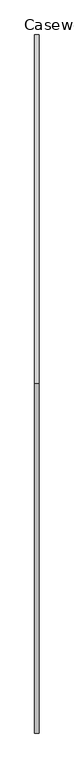
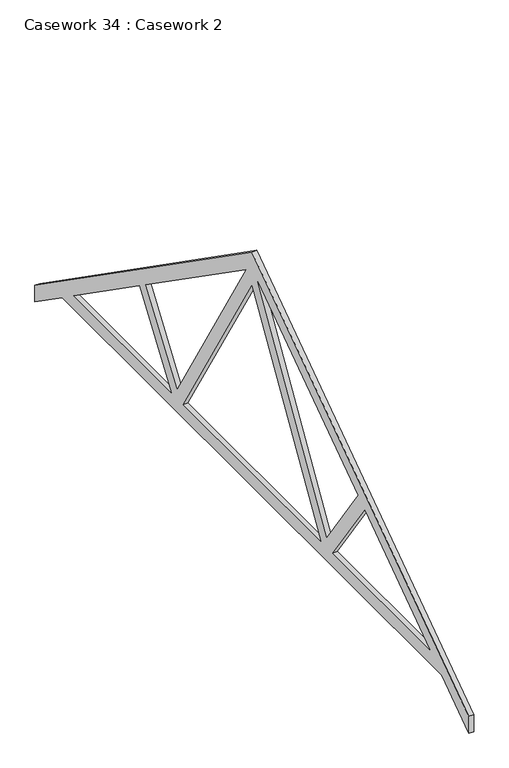
"""IFC4 building model written with IfcOpenShell, lengths in millimetres: furniture geometry, Casework 34 : Casework 2."""

from ifc_helpers import new_model, si_unit, frame, origin, place, context, project, spatial, polyline, outline, extrude, source, transform, mapped, element, save


def casework_34_casework_2_77ddbc4c(model_context):
    return source(origin(), model_context, "Body", "SweptSolid", [
        extrude(outline(polyline([(6583.1149316, 5285.0), (-277.3850684, 5285.0), (-767.3850684, 4941.8983063), (-767.3850684, 5125.0144946), (3152.8649316, 7870.0030963), (7073.1149316, 5125.0144946), (7073.1149316, 4941.8983063), (6583.1149316, 5285.0)]), holes=[polyline([(4612.3149663, 5435.0), (6368.8927306, 5435.0), (5190.2113591, 6260.3215815), (4612.3149663, 5435.0)]), polyline([(4394.2037684, 5435.0), (3152.8649316, 7500.9347567), (1911.5260948, 5435.0), (4394.2037684, 5435.0)]), polyline([(4504.5438357, 5542.6038939), (5067.3385525, 6346.3580469), (3262.0771677, 7610.415677), (4504.5438357, 5542.6038939)]), polyline([(1693.4148969, 5435.0), (1115.5185041, 6260.3215815), (-63.1628674, 5435.0), (1693.4148969, 5435.0)]), polyline([(1801.1860276, 5542.6038939), (3043.6526956, 7610.415677), (1238.3913108, 6346.3580469), (1801.1860276, 5542.6038939)])]), frame((-4421.5247381, 0.0, 0.0), z_axis=(1.0, 0.0, 0.0), x_axis=(0.0, 1.0, 0.0)), (0.0, 0.0, 1.0), 49.6351915),
    ])


if __name__ == "__main__":
    model = new_model("IFC4")
    model_context = context("Model", 3, world=origin())
    ifc_project = project(units=[si_unit("LENGTHUNIT", "METRE", prefix="MILLI")], contexts=[model_context])
    site = spatial("IfcSite", under=ifc_project)
    building = spatial("IfcBuilding", under=site)
    placement = place(None, origin())
    casework_34_casework_2_shape = casework_34_casework_2_77ddbc4c(model_context)
    element("IfcFurniture", 1, ObjectType="Casework 34 : Casework 2", at=placement, inside=building, context=model_context, shape_type="MappedRepresentation", body=[
        mapped(casework_34_casework_2_shape, transform((0.0, 0.0, 0.0), x_axis=(1.0, 0.0, 0.0), y_axis=(0.0, 1.0, 0.0), z_axis=(0.0, 0.0, 1.0))),
    ])
    save(model, "model.ifc")
